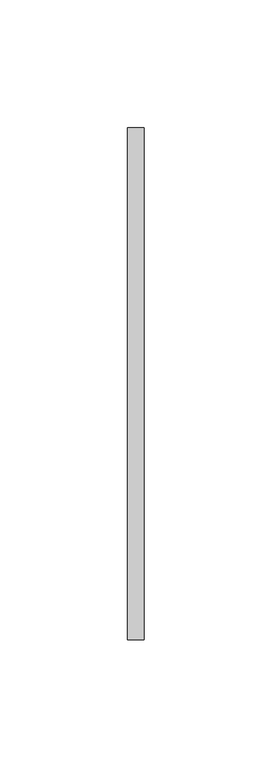
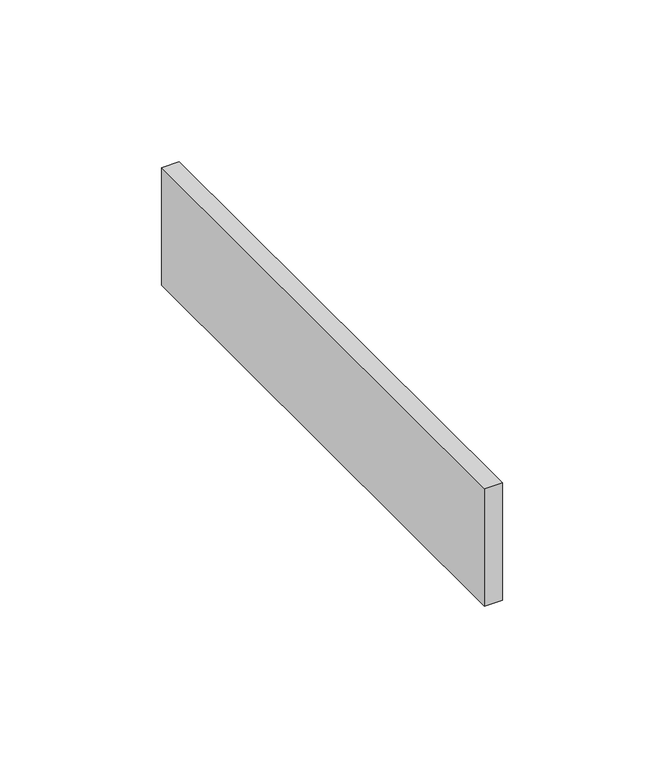
"""IFC4 building model written with IfcOpenShell, lengths in millimetres: proxy geometry, Inner panel1:Inner panel:306176:Inner panel:306176 : Inner panel1:Inner panel:306176:300391:Inner panel:306176:Inner panel:306176 : Inner panel1:Inner panel:306176:300391 : Inner panel1:Inner panel:306176:Inner panel:306176 : Inner panel1:Inner panel:306176:300391:1 : Inner panel1:Inner panel:306176:Inner panel:306176 : Inner panel1:Inner panel:306176:300391:Inner panel:306176:Inner panel:306176 : Inner panel1:Inner panel:306176:300391 : Inner panel1:Inner panel:306176:Inner panel:306176 : Inner panel1:Inner panel:306176:300391:300168."""

from ifc_helpers import new_model, si_unit, origin, origin_with_axes, place, context, project, spatial, polyline, outline, extrude, source, transform, mapped, element, save


def generic_models_46ba5da4(model_context):
    return source(origin(), model_context, "Body", "SweptSolid", [
        extrude(outline(polyline([(593757.1367239, -578997.5163841), (593750.7867239, -578997.5163841), (593750.7867239, -578797.4913841), (593757.1367239, -578797.4913841), (593757.1367239, -578997.5163841)])), origin_with_axes(), (0.0, 0.0, 1.0), 44.45),
    ])


if __name__ == "__main__":
    model = new_model("IFC4")
    model_context = context("Model", 3, world=origin())
    ifc_project = project(units=[si_unit("LENGTHUNIT", "METRE", prefix="MILLI")], contexts=[model_context])
    site = spatial("IfcSite", under=ifc_project)
    building = spatial("IfcBuilding", under=site)
    placement = place(None, origin())
    generic_models_shape = generic_models_46ba5da4(model_context)
    element("IfcBuildingElementProxy", 1, Name="Inner panel1:Inner panel:306176:Inner panel:306176 : Inner panel1:Inner panel:306176:300391:Inner panel:306176:Inner panel:306176 : Inner panel1:Inner panel:306176:300391 : Inner panel1:Inner panel:306176:Inner panel:306176 : Inner panel1:Inner panel:306176:300391:1 : Inner panel1:Inner panel:306176:Inner panel:306176 : Inner panel1:Inner panel:306176:300391:Inner panel:306176:Inner panel:306176 : Inner panel1:Inner panel:306176:300391 : Inner panel1:Inner panel:306176:Inner panel:306176 : Inner panel1:Inner panel:306176:300391:300168", ObjectType="Inner panel1:Inner panel:306176:Inner panel:306176 : Inner panel1:Inner panel:306176:300391:Inner panel:306176:Inner panel:306176 : Inner panel1:Inner panel:306176:300391 : Inner panel1:Inner panel:306176:Inner panel:306176 : Inner panel1:Inner panel:306176:300391:1 : Inner panel1:Inner panel:306176:Inner panel:306176 : Inner panel1:Inner panel:306176:300391:Inner panel:306176:Inner panel:306176 : Inner panel1:Inner panel:306176:300391 : Inner panel1:Inner panel:306176:Inner panel:306176 : Inner panel1:Inner panel:306176:300391:300168", at=placement, inside=building, context=model_context, shape_type="MappedRepresentation", body=[
        mapped(generic_models_shape, transform((0.0, 0.0, 0.0), x_axis=(1.0, 0.0, 0.0), y_axis=(0.0, 1.0, 0.0), z_axis=(0.0, 0.0, 1.0))),
    ])
    save(model, "model.ifc")

# Revit data of these elements
# Type "Inner panel1:Inner panel:306176:Inner panel:306176 : Inner panel1:Inner panel:306176:300391:Inner panel:306176:Inner panel:306176 : Inner panel1:Inner panel:306176:300391 : Inner panel1:Inner panel:306176:Inner panel:306176 : Inner panel1:Inner panel:306176:300391:1 : Inner panel1:Inner panel:306176:Inner panel:306176 : Inner panel1:Inner panel:306176:300391:Inner panel:306176:Inner panel:306176 : Inner panel1:Inner panel:306176:300391 : Inner panel1:Inner panel:306176:Inner panel:306176 : Inner panel1:Inner panel:306176:300391:300168"
#   NameOverride = "Inner panel1:Inner panel:306176:Inner panel:306176 : Inner panel1:Inner panel:306176:300391:Inner panel:306176:Inner panel:306176 : Inner panel1:Inner panel:306176:300391 : Inner panel1:Inner panel:306176:Inner panel:306176 : Inner panel1:Inner panel:306176:300391:300168"
#   ObjectTypeOverride = "Inner panel:306176:Inner panel:306176 : Inner panel1:Inner panel:306176:300391 : Inner panel1:Inner panel:306176:Inner panel:306176 : Inner panel1:Inner panel:306176:300391"
#   Reference = "Inner panel"
#   Tag = "300168"
# Element 1 (IfcBuildingElementProxy, "Inner panel1:Inner panel:306176:Inner panel:306176 : Inner panel1:Inner panel:306176:300391:Inner panel:306176:Inner panel:306176 : Inner panel1:Inner panel:306176:300391 : Inner panel1:Inner panel:306176:Inner panel:306176 : Inner panel1:Inner panel:306176:300391:1 : Inner panel1:Inner panel:306176:Inner panel:306176 : Inner panel1:Inner panel:306176:300391:Inner panel:306176:Inner panel:306176 : Inner panel1:Inner panel:306176:300391 : Inner panel1:Inner panel:306176:Inner panel:306176 : Inner panel1:Inner panel:306176:300391:300168")
#   Materials on its faces: "STEEL END CAP AT BASE CHANNEL - PAINT TO MATCH STRUCT. STEEL"
# Materials
#   "STEEL END CAP AT BASE CHANNEL - PAINT TO MATCH STRUCT. STEEL": class "Generic", colour RGB 120 120 120, transparency 0, Cost = 0
